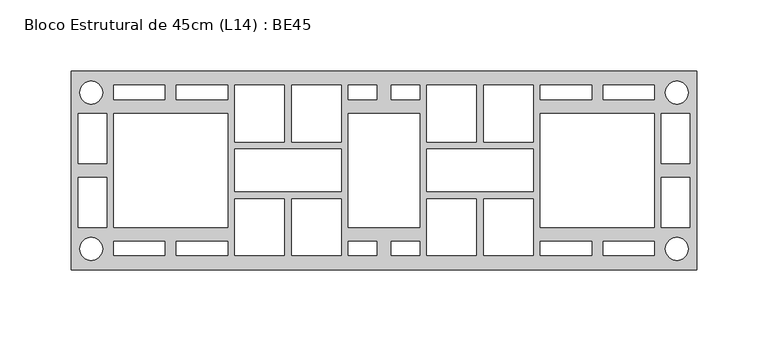
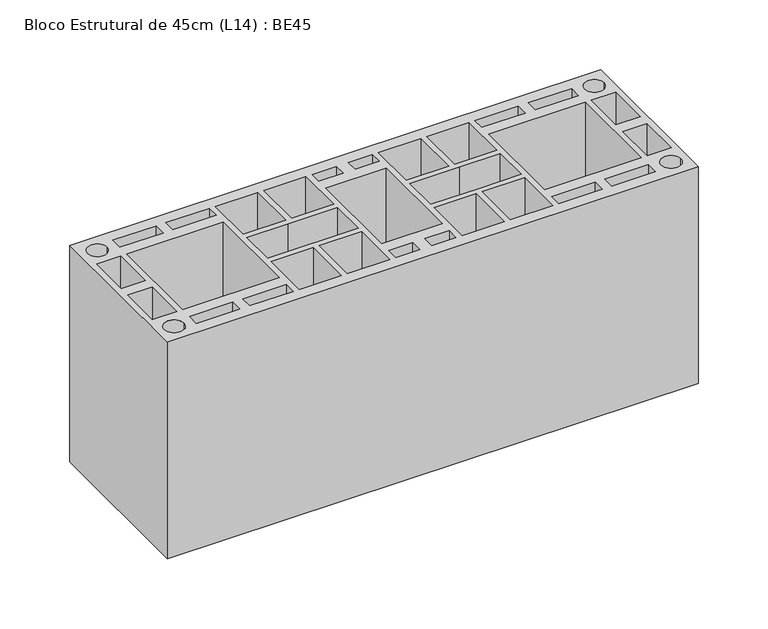
"""IFC4 building model written with IfcOpenShell, lengths in millimetres: proxy geometry, Bloco Estrutural de 45cm (L14) : BE45."""

from ifc_helpers import new_model, si_unit, point, frame_2d, origin, origin_with_axes, place, context, project, spatial, polyline, circle_curve, trimmed, segment, composite_curve, outline, extrude, source, transform, mapped, element, save


def bloco_estrutural_de_45cm_l14_be45_067f568e(model_context):
    return source(origin(), model_context, "Body", "SweptSolid", [
        extrude(outline(polyline([(440.0, 0.0), (0.0, 0.0), (0.0, 140.0), (440.0, 140.0), (440.0, 0.0)]), holes=[composite_curve([segment(trimmed(circle_curve(frame_2d((14.1087523, 124.7509514)), 8.0), [point((6.1087523, 124.7509514))], [point((22.1087523, 124.7509514))], True, "CARTESIAN"), True, "CONTINUOUS"), segment(trimmed(circle_curve(frame_2d((14.1087523, 124.7509514)), 8.0), [point((22.1087523, 124.7509514))], [point((6.1087523, 124.7509514))], True, "CARTESIAN"), True, "CONTINUOUS")], self_intersect=False), composite_curve([segment(trimmed(circle_curve(frame_2d((14.1087523, 14.7509514)), 8.0), [point((6.1087523, 14.7509514))], [point((22.1087523, 14.7509514))], True, "CARTESIAN"), True, "CONTINUOUS"), segment(trimmed(circle_curve(frame_2d((14.1087523, 14.7509514)), 8.0), [point((22.1087523, 14.7509514))], [point((6.1087523, 14.7509514))], True, "CARTESIAN"), True, "CONTINUOUS")], self_intersect=False), polyline([(110.0, 110.0), (30.0, 110.0), (30.0, 30.0), (110.0, 30.0), (110.0, 110.0)]), polyline([(245.0, 110.0), (195.0, 110.0), (195.0, 30.0), (245.0, 30.0), (245.0, 110.0)]), polyline([(66.0, 130.0), (30.0, 130.0), (30.0, 120.0), (66.0, 120.0), (66.0, 130.0)]), polyline([(66.0, 20.0), (30.0, 20.0), (30.0, 10.0), (66.0, 10.0), (66.0, 20.0)]), polyline([(74.0, 130.0), (74.0, 120.0), (110.0, 120.0), (110.0, 130.0), (74.0, 130.0)]), polyline([(74.0, 20.0), (74.0, 10.0), (110.0, 10.0), (110.0, 20.0), (74.0, 20.0)]), composite_curve([segment(trimmed(circle_curve(frame_2d((425.8912477, 124.7509514)), 8.0), [point((433.8912477, 124.7509514))], [point((417.8912477, 124.7509514))], True, "CARTESIAN"), True, "CONTINUOUS"), segment(trimmed(circle_curve(frame_2d((425.8912477, 124.7509514)), 8.0), [point((417.8912477, 124.7509514))], [point((433.8912477, 124.7509514))], True, "CARTESIAN"), True, "CONTINUOUS")], self_intersect=False), composite_curve([segment(trimmed(circle_curve(frame_2d((425.8912477, 14.7509514)), 8.0), [point((433.8912477, 14.7509514))], [point((417.8912477, 14.7509514))], True, "CARTESIAN"), True, "CONTINUOUS"), segment(trimmed(circle_curve(frame_2d((425.8912477, 14.7509514)), 8.0), [point((417.8912477, 14.7509514))], [point((433.8912477, 14.7509514))], True, "CARTESIAN"), True, "CONTINUOUS")], self_intersect=False), polyline([(330.0, 110.0), (330.0, 30.0), (410.0, 30.0), (410.0, 110.0), (330.0, 110.0)]), polyline([(374.0, 130.0), (374.0, 120.0), (410.0, 120.0), (410.0, 130.0), (374.0, 130.0)]), polyline([(374.0, 20.0), (374.0, 10.0), (410.0, 10.0), (410.0, 20.0), (374.0, 20.0)]), polyline([(366.0, 130.0), (330.0, 130.0), (330.0, 120.0), (366.0, 120.0), (366.0, 130.0)]), polyline([(366.0, 20.0), (330.0, 20.0), (330.0, 10.0), (366.0, 10.0), (366.0, 20.0)]), polyline([(25.0, 110.0), (5.0, 110.0), (5.0, 75.0), (25.0, 75.0), (25.0, 110.0)]), polyline([(25.0, 30.0), (25.0, 65.0), (5.0, 65.0), (5.0, 30.0), (25.0, 30.0)]), polyline([(415.0, 110.0), (415.0, 75.0), (435.0, 75.0), (435.0, 110.0), (415.0, 110.0)]), polyline([(415.0, 30.0), (435.0, 30.0), (435.0, 65.0), (415.0, 65.0), (415.0, 30.0)]), polyline([(225.0, 20.0), (225.0, 10.0), (245.0, 10.0), (245.0, 20.0), (225.0, 20.0)]), polyline([(215.0, 20.0), (195.0, 20.0), (195.0, 10.0), (215.0, 10.0), (215.0, 20.0)]), polyline([(225.0, 120.0), (245.0, 120.0), (245.0, 130.0), (225.0, 130.0), (225.0, 120.0)]), polyline([(215.0, 120.0), (215.0, 130.0), (195.0, 130.0), (195.0, 120.0), (215.0, 120.0)]), polyline([(150.0, 130.0), (115.0, 130.0), (115.0, 90.0), (150.0, 90.0), (150.0, 130.0)]), polyline([(190.0, 130.0), (155.0, 130.0), (155.0, 90.0), (190.0, 90.0), (190.0, 130.0)]), polyline([(115.0, 85.0), (115.0, 55.0), (190.0, 55.0), (190.0, 85.0), (148.9828076, 85.0), (115.0, 85.0)]), polyline([(155.0, 50.0), (155.0, 10.0), (190.0, 10.0), (190.0, 50.0), (155.0, 50.0)]), polyline([(150.0, 10.0), (150.0, 50.0), (115.0, 50.0), (115.0, 10.0), (150.0, 10.0)]), polyline([(290.0, 130.0), (290.0, 90.0), (325.0, 90.0), (325.0, 130.0), (290.0, 130.0)]), polyline([(250.0, 130.0), (250.0, 90.0), (285.0, 90.0), (285.0, 130.0), (250.0, 130.0)]), polyline([(325.0, 85.0), (291.0171924, 85.0), (250.0, 85.0), (250.0, 55.0), (291.0171924, 55.0), (325.0, 55.0), (325.0, 85.0)]), polyline([(285.0, 50.0), (250.0, 50.0), (250.0, 10.0), (285.0, 10.0), (285.0, 50.0)]), polyline([(290.0, 10.0), (325.0, 10.0), (325.0, 50.0), (290.0, 50.0), (290.0, 10.0)])]), origin_with_axes(), (0.0, 0.0, 1.0), 190.0),
    ])


if __name__ == "__main__":
    model = new_model("IFC4")
    model_context = context("Model", 3, world=origin())
    ifc_project = project(units=[si_unit("LENGTHUNIT", "METRE", prefix="MILLI")], contexts=[model_context])
    site = spatial("IfcSite", under=ifc_project)
    building = spatial("IfcBuilding", under=site)
    placement = place(None, origin())
    bloco_estrutural_de_45cm_l14_be45_shape = bloco_estrutural_de_45cm_l14_be45_067f568e(model_context)
    element("IfcBuildingElementProxy", 1, Name="Bloco Estrutural de 45cm (L14) : BE45", ObjectType="Bloco Estrutural de 45cm (L14) : BE45", at=placement, inside=building, context=model_context, shape_type="MappedRepresentation", body=[
        mapped(bloco_estrutural_de_45cm_l14_be45_shape, transform((0.0, 0.0, 0.0), x_axis=(1.0, 0.0, 0.0), y_axis=(0.0, 1.0, 0.0), z_axis=(0.0, 0.0, 1.0))),
    ])
    save(model, "model.ifc")

# Revit data of these elements
# Project information
#   Project Issue Date = "Data de emissão"
#   Project Status = "Status do projeto"
#   Client Name = "Proprietário"
#   Project Address = "Insira aqui o endereço"
#   Project Name = "Nome do projeto"
#   Project Number = "0001"
# Type "Bloco Estrutural de 45cm (L14) : BE45"
#   Material [instance default] = Blocos Cerâmicos
#   Default Elevation = 0
# Element 1 (IfcBuildingElementProxy, "Bloco Estrutural de 45cm (L14) : BE45")
#   Materials on its faces: "Blocos Cerâmicos"
# Materials
#   "Blocos Cerâmicos": class "Genérico", colour RGB 177 84 47, transparency 0, Cost = 0
